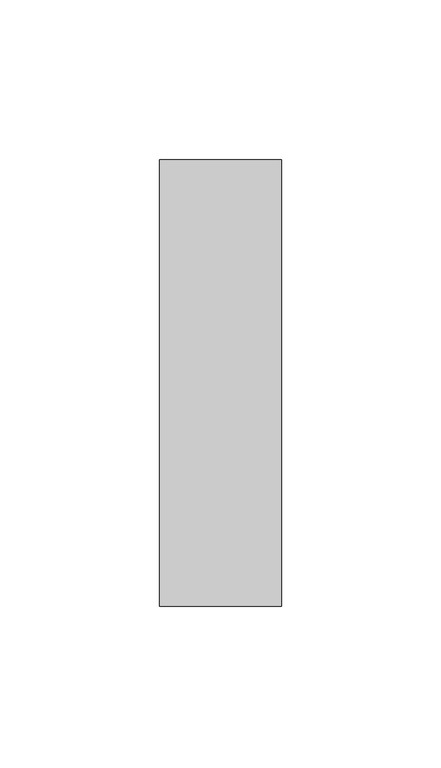
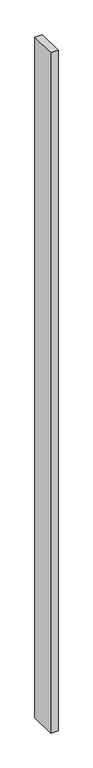
"""IFC4 building model written with IfcOpenShell, lengths in millimetres: proxy geometry, Generic Models 2:Generic Models 2:310765:Generic Models 2:310765 : Generic Models 2:Generic Models 2:310765:66 : Generic Models 2:Generic Models 2:310765:Generic Models 2:310765 : Generic Models 2:Generic Models 2:310765:300385."""

from ifc_helpers import new_model, si_unit, frame, origin, place, context, project, spatial, polyline, outline, extrude, source, transform, mapped, element, save


def generic_models_5a7814f5(model_context):
    return source(origin(), model_context, "Body", "SweptSolid", [
        extrude(outline(polyline([(578685.4117239, -568215.2163841), (578647.3117239, -568215.2163841), (578647.3117239, -568075.5163841), (578685.4117239, -568075.5163841), (578685.4117239, -568215.2163841)])), frame((0.0, 0.0, 4860.0679991), z_axis=(0.0, 0.0, 1.0), x_axis=(1.0, 0.0, 0.0)), (0.0, 0.0, 1.0), 3695.7),
    ])


if __name__ == "__main__":
    model = new_model("IFC4")
    model_context = context("Model", 3, world=origin())
    ifc_project = project(units=[si_unit("LENGTHUNIT", "METRE", prefix="MILLI")], contexts=[model_context])
    site = spatial("IfcSite", under=ifc_project)
    building = spatial("IfcBuilding", under=site)
    placement = place(None, origin())
    generic_models_shape = generic_models_5a7814f5(model_context)
    element("IfcBuildingElementProxy", 1, Name="Generic Models 2:Generic Models 2:310765:Generic Models 2:310765 : Generic Models 2:Generic Models 2:310765:66 : Generic Models 2:Generic Models 2:310765:Generic Models 2:310765 : Generic Models 2:Generic Models 2:310765:300385", ObjectType="Generic Models 2:Generic Models 2:310765:Generic Models 2:310765 : Generic Models 2:Generic Models 2:310765:66 : Generic Models 2:Generic Models 2:310765:Generic Models 2:310765 : Generic Models 2:Generic Models 2:310765:300385", at=placement, inside=building, context=model_context, shape_type="MappedRepresentation", body=[
        mapped(generic_models_shape, transform((0.0, 0.0, 0.0), x_axis=(1.0, 0.0, 0.0), y_axis=(0.0, 1.0, 0.0), z_axis=(0.0, 0.0, 1.0))),
    ])
    save(model, "model.ifc")

# Revit data of these elements
# Type "Generic Models 2:Generic Models 2:310765:Generic Models 2:310765 : Generic Models 2:Generic Models 2:310765:66 : Generic Models 2:Generic Models 2:310765:Generic Models 2:310765 : Generic Models 2:Generic Models 2:310765:300385"
#   NameOverride = "Generic Models 2:Generic Models 2:310765:Generic Models 2:310765 : Generic Models 2:Generic Models 2:310765:300385"
#   ObjectTypeOverride = "Generic Models 2:310765 : Generic Models 2:Generic Models 2:310765"
#   Reference = "Generic Models 2"
#   Tag = "300385"
# Element 1 (IfcBuildingElementProxy, "Generic Models 2:Generic Models 2:310765:Generic Models 2:310765 : Generic Models 2:Generic Models 2:310765:66 : Generic Models 2:Generic Models 2:310765:Generic Models 2:310765 : Generic Models 2:Generic Models 2:310765:300385")
#   Materials on its faces: "BLOCKING - SIZE AS NEC."
# Materials
#   "BLOCKING - SIZE AS NEC.": class "Wood", colour RGB 144 113 62, transparency 0, Description = "Pinus Echinata", Cost = 0
